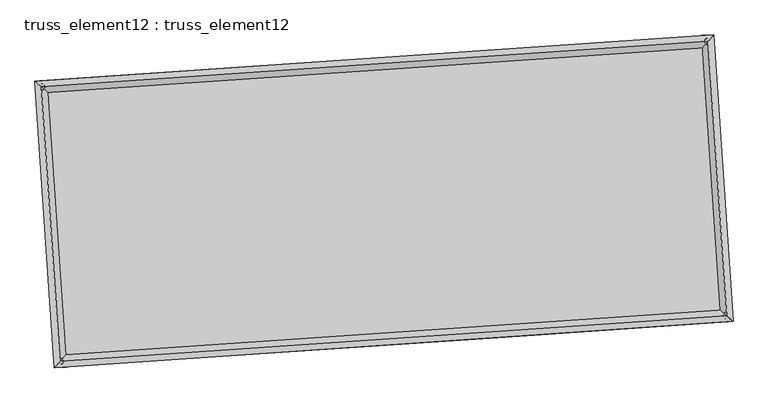
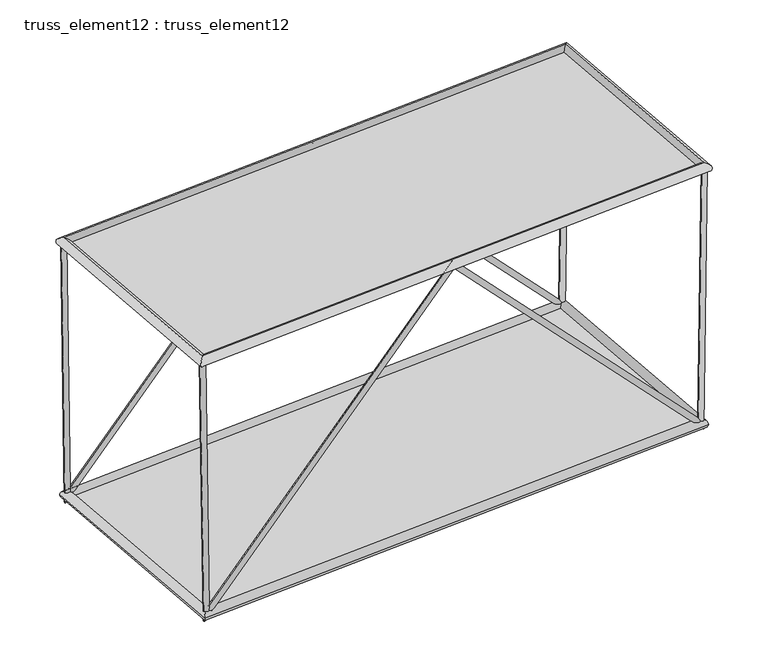
"""IFC4 building model written with IfcOpenShell, lengths in millimetres: plate geometry, truss_element12 : truss_element12."""

import ifcopenshell
import ifcopenshell.guid

model = None  # the IFC model being written
_history = None  # IfcOwnerHistory: only IFC2X3 demands one
_inside = {}  # id of a spatial element -> (the spatial element, [elements in it])
_under = {}  # id of a project, library or spatial element -> (it, [spatial elements below it])
_declared = {}  # id of a project -> (the project, [libraries it declares])
_typed = {}  # id of a type object -> (the type object, [elements of that type])
_made_of = {}  # id of a material, layer set ... -> (it, [elements and type objects made of it])


def new_model(schema):
    """Start an empty IFC model of exactly this schema.

    Asked for "IFC4X3", IfcOpenShell would pick the latest addendum, in which some entities
    have other attributes; the version numbers below select the first issue.
    IFC2X3 requires an IfcOwnerHistory on every rooted entity: one is made here for all.
    """
    global model, _history
    if schema == "IFC4X3":
        model = ifcopenshell.file(schema_version=(4, 3, 0, 0))
    else:
        model = ifcopenshell.file(schema=schema)
    _inside.clear()
    _under.clear()
    _declared.clear()
    _typed.clear()
    _made_of.clear()
    _history = None
    if model.schema == "IFC2X3":
        org = make("IfcOrganization", Name="unknown")
        user = make(
            "IfcPersonAndOrganization",
            ThePerson=make("IfcPerson", FamilyName="unknown"),
            TheOrganization=org,
        )
        app = make(
            "IfcApplication",
            ApplicationDeveloper=org,
            Version="unknown",
            ApplicationFullName="unknown",
            ApplicationIdentifier="unknown",
        )
        _history = make(
            "IfcOwnerHistory",
            OwningUser=user,
            OwningApplication=app,
            ChangeAction="ADDED",
            CreationDate=0,
        )
    return model


def make(cls, **values):
    """One entity of the class cls with the attributes given. An attribute that is None is left unset."""
    return model.create_entity(
        cls, **{name: value for name, value in values.items() if value is not None}
    )


def rooted(cls, **values):
    """An entity with a GlobalId (a new one), such as an element, a storey or a relation."""
    return make(cls, GlobalId=ifcopenshell.guid.new(), OwnerHistory=_history, **values)


def si_unit(unit_type, name, prefix=None):
    """IfcSIUnit, for example si_unit("LENGTHUNIT", "METRE", prefix="MILLI")."""
    return make("IfcSIUnit", UnitType=unit_type, Prefix=prefix, Name=name)


def assignment(units):
    """IfcUnitAssignment: the units of a project."""
    return None if units is None else make("IfcUnitAssignment", Units=units)


def point(xyz):
    """IfcCartesianPoint."""
    return None if xyz is None else make("IfcCartesianPoint", Coordinates=xyz)


def direction(xyz):
    """IfcDirection."""
    return None if xyz is None else make("IfcDirection", DirectionRatios=xyz)


def frame(location, z_axis=None, x_axis=None):
    """IfcAxis2Placement3D, a coordinate frame: its origin and axes. An axis left out is left unset."""
    return make(
        "IfcAxis2Placement3D",
        Location=point(location),
        Axis=direction(z_axis),
        RefDirection=direction(x_axis),
    )


def origin():
    """The frame at (0, 0, 0) with its axes left unset."""
    return frame((0.0, 0.0, 0.0))


def origin_with_axes():
    """The frame at (0, 0, 0) with the z axis (0, 0, 1) and the x axis (1, 0, 0) written out."""
    return frame((0.0, 0.0, 0.0), z_axis=(0.0, 0.0, 1.0), x_axis=(1.0, 0.0, 0.0))


def place(relative_to, where):
    """IfcLocalPlacement: puts the frame where relative to a parent placement (None: the world)."""
    return make(
        "IfcLocalPlacement", PlacementRelTo=relative_to, RelativePlacement=where
    )


def context(
    kind, dimensions, precision=None, world=None, true_north=None, identifier=None
):
    """IfcGeometricRepresentationContext, for example the 3D "Model" context."""
    return make(
        "IfcGeometricRepresentationContext",
        ContextIdentifier=identifier,
        ContextType=kind,
        CoordinateSpaceDimension=dimensions,
        Precision=precision,
        WorldCoordinateSystem=world,
        TrueNorth=true_north,
    )


def project(units=None, contexts=None):
    """IfcProject with its units and contexts."""
    return rooted(
        "IfcProject",
        Name="project",
        RepresentationContexts=contexts,
        UnitsInContext=assignment(units),
    )


def spatial(cls, under=None, at=None, **own):
    """A site, building, storey or space (cls), placed at a placement, below another one or the project."""
    s = rooted(cls, ObjectPlacement=at, **own)
    if under is not None:
        _under.setdefault(under.id(), (under, []))[1].append(s)
    return s


def polyline(points):
    """IfcPolyline through the points."""
    return make("IfcPolyline", Points=[point(p) for p in points])


def circle_curve(where, radius):
    """IfcCircle in the frame where."""
    return make("IfcCircle", Position=where, Radius=radius)


def ellipse_curve(where, semi_axis1, semi_axis2):
    """IfcEllipse in the frame where."""
    return make(
        "IfcEllipse", Position=where, SemiAxis1=semi_axis1, SemiAxis2=semi_axis2
    )


def outline(outer, holes=None, kind="AREA"):
    """IfcArbitraryClosedProfileDef: a profile drawn as a closed curve; with holes, ...WithVoids."""
    if holes is None:
        return make("IfcArbitraryClosedProfileDef", ProfileType=kind, OuterCurve=outer)
    return make(
        "IfcArbitraryProfileDefWithVoids",
        ProfileType=kind,
        OuterCurve=outer,
        InnerCurves=holes,
    )


def extrude(swept, where, along, depth):
    """IfcExtrudedAreaSolid: the profile swept, set in the frame where, extruded along a direction by depth."""
    return make(
        "IfcExtrudedAreaSolid",
        SweptArea=swept,
        Position=where,
        ExtrudedDirection=direction(along),
        Depth=depth,
    )


def shape(context_of_items, identifier, shape_type, items):
    """IfcShapeRepresentation: the items that make up one representation, for example the "Body"."""
    return make(
        "IfcShapeRepresentation",
        ContextOfItems=context_of_items,
        RepresentationIdentifier=identifier,
        RepresentationType=shape_type,
        Items=items,
    )


def source(mapping_origin, context_of_items, identifier, shape_type, items):
    """IfcRepresentationMap: a shape defined once, which mapped items show again and again."""
    return make(
        "IfcRepresentationMap",
        MappingOrigin=mapping_origin,
        MappedRepresentation=shape(context_of_items, identifier, shape_type, items),
    )


def transform(
    local_origin,
    x_axis=None,
    y_axis=None,
    z_axis=None,
    scale=None,
    scale2=None,
    scale3=None,
    uniform=True,
):
    """IfcCartesianTransformationOperator3D, or its non-uniform kind. x_axis, y_axis, z_axis: its Axis1, 2, 3."""
    if uniform:
        return make(
            "IfcCartesianTransformationOperator3D",
            Axis1=direction(x_axis),
            Axis2=direction(y_axis),
            LocalOrigin=point(local_origin),
            Scale=scale,
            Axis3=direction(z_axis),
        )
    return make(
        "IfcCartesianTransformationOperator3DnonUniform",
        Axis1=direction(x_axis),
        Axis2=direction(y_axis),
        LocalOrigin=point(local_origin),
        Scale=scale,
        Axis3=direction(z_axis),
        Scale2=scale2,
        Scale3=scale3,
    )


def mapped(mapping_source, mapping_target):
    """IfcMappedItem: shows the shape of a source again, moved by a transform."""
    return make(
        "IfcMappedItem", MappingSource=mapping_source, MappingTarget=mapping_target
    )


def made_of(thing, what):
    """Note that an element or type object is made of a material, layer set ...; save() writes the relation."""
    if what is not None:
        _made_of.setdefault(what.id(), (what, []))[1].append(thing)
    return thing


def element(
    cls,
    number,
    at=None,
    inside=None,
    cuts=None,
    type_object=None,
    material=None,
    context=None,
    identifier="Body",
    shape_type=None,
    held_by="IfcProductDefinitionShape",
    body=None,
    shapes=None,
    **own,
):
    """One element of the class cls, such as IfcWall. Its Tag is "e" and its number.

    at: its placement. inside: the storey or other place that contains it. cuts: it is an
    opening in that element (IfcRelVoidsElement). A single representation is given by context,
    identifier, shape_type and body (its items); several are given by shapes. held_by: the class
    of the entity that holds the representations. save() writes the other relations.
    """
    e = rooted(cls, Tag="e%d" % number, ObjectPlacement=at, **own)
    if body is not None:
        shapes = [shape(context, identifier, shape_type, body)]
    if shapes is not None:
        e.Representation = make(held_by, Representations=shapes)
    if inside is not None:
        _inside.setdefault(inside.id(), (inside, []))[1].append(e)
    if cuts is not None:
        rooted(
            "IfcRelVoidsElement", RelatingBuildingElement=cuts, RelatedOpeningElement=e
        )
    if type_object is not None:
        _typed.setdefault(type_object.id(), (type_object, []))[1].append(e)
    return made_of(e, material)


def aggregate(whole, parts):
    """IfcRelAggregates: a whole, such as a stair, and the parts it consists of."""
    return rooted("IfcRelAggregates", RelatingObject=whole, RelatedObjects=parts)


def save(model, path):
    """Write the relations noted so far, then the file.

    IfcRelAggregates (storeys below a building ...), IfcRelContainedInSpatialStructure (elements
    in a storey), IfcRelDefinesByType, IfcRelAssociatesMaterial and IfcRelDeclares: one each for
    every whole, place, type object, material and project.
    """
    for whole, parts in _under.values():
        aggregate(whole, parts)
    for where, things in _inside.values():
        rooted(
            "IfcRelContainedInSpatialStructure",
            RelatedElements=things,
            RelatingStructure=where,
        )
    for kind, things in _typed.values():
        rooted("IfcRelDefinesByType", RelatedObjects=things, RelatingType=kind)
    for what, things in _made_of.values():
        rooted("IfcRelAssociatesMaterial", RelatedObjects=things, RelatingMaterial=what)
    for by, libraries in _declared.values():
        rooted("IfcRelDeclares", RelatingContext=by, RelatedDefinitions=libraries)
    model.write(path)


def plane_surface(at):
    """IfcPlane: the flat surface through the origin of the frame at, square to its z axis."""
    return make("IfcPlane", Position=at)


def cylinder_surface(at, radius):
    """IfcCylindricalSurface: all points at the distance radius from the z axis of the frame at."""
    return make("IfcCylindricalSurface", Position=at, Radius=radius)


def advanced_brep(points, edges, surfaces, faces):
    """IfcAdvancedBrep: a solid bounded by faces that lie on surfaces and meet in shared edges.

    An edge is (start, end): straight between two places in points (the first is 0);
    or (start, end, curve); or (start, end, curve, False) where it runs against its curve.
    A face is (place in surfaces, loops), or (place, loops, False) where it looks against
    its surface's normal. A loop lists edges by number (the first is 1), with a minus sign
    where the edge is run from its end to its start. The first loop is the outer one.
    """
    corners = [point(p) for p in points]
    vertices = [make("IfcVertexPoint", VertexGeometry=c) for c in corners]
    made = []
    for start, end, *more in edges:
        made.append(
            make(
                "IfcEdgeCurve",
                EdgeStart=vertices[start],
                EdgeEnd=vertices[end],
                EdgeGeometry=more[0] if more else make("IfcPolyline", Points=[corners[start], corners[end]]),
                SameSense=more[1] if len(more) > 1 else True,
            )
        )
    hull = []
    for where, loops, *sense in faces:
        bounds = []
        for j, loop in enumerate(loops):
            ring = [make("IfcOrientedEdge", EdgeElement=made[abs(k) - 1], Orientation=k > 0) for k in loop]
            bounds.append(
                make(
                    "IfcFaceOuterBound" if j == 0 else "IfcFaceBound",
                    Bound=make("IfcEdgeLoop", EdgeList=ring),
                    Orientation=True,
                )
            )
        hull.append(make("IfcAdvancedFace", Bounds=bounds, FaceSurface=surfaces[where], SameSense=sense[0] if sense else True))
    return make("IfcAdvancedBrep", Outer=make("IfcClosedShell", CfsFaces=hull))


def truss_element12_truss_element12_be2aad90(model_context):
    return source(origin(), model_context, "Body", "SolidModel", [
        advanced_brep(
        [(-3735.6006401, 2271.406017, 5000.2050975), (-3834.6940161, 2258.0454232, 4998.791816), (-3666.6666291, 2276.1063651, 122.4057611), (-3762.3202537, 2262.980315, -122.4057611), (1063.0860418, 2598.6102203, 5071.6275519), (1063.5437029, 2592.0376334, 4927.3870537), (5794.0749811, 2921.1983719, 122.4145359), (5890.6859959, 2921.1821166, -122.4145359), (5861.782005, 2925.8150565, 5000.2102148), (5961.7721407, 2926.0292106, 4998.822083)],
        [
            (0, 1, circle_curve(frame((-3785.1473281, 2264.7257201, 4999.4984567), z_axis=(-0.014130777343730014, -0.0009635239909554328, 0.9998996913456774), x_axis=(-0.13360615268411807, 0.9910340686191066, -0.0009331672991190194)), 50.0)),
            (1, 0, circle_curve(frame((-3785.1473281, 2264.7257201, 4999.4984567), z_axis=(-0.014130777343730014, -0.0009635239909554328, 0.9998996913456774), x_axis=(-0.13360615268411807, 0.9910340686191066, -0.0009331672991190194)), 50.0)),
            (0, 2),
            (2, 3, ellipse_curve(frame((-3714.4934414, 2269.54334, 0.0), z_axis=(-0.9284028499826127, -0.06330426115068324, 0.366143030336955), x_axis=(0.3652948219557198, 0.024908065293541812, 0.9305585856546978)), 131.8265203, 50.0)),
            (3, 1),
            (3, 2, ellipse_curve(frame((-3714.4934414, 2269.54334, 0.0), z_axis=(-0.9284028499826127, -0.06330426115068324, 0.366143030336955), x_axis=(0.3652948219557198, 0.024908065293541812, 0.9305585856546978)), 131.8265203, 50.0)),
            (2, 4),
            (4, 5, ellipse_curve(frame((1063.3148723, 2595.3239268, 4999.5073028), z_axis=(-0.9976833939203528, -0.06802823808179481, -6.571949967975178e-05), x_axis=(6.556725362871375e-05, 4.470781780485672e-06, -0.9999999978404738)), 72.2772914, 50.0)),
            (5, 3),
            (5, 4, ellipse_curve(frame((1063.3148723, 2595.3239268, 4999.5073028), z_axis=(-0.9976833939203528, -0.06802823808179481, -6.571949967975178e-05), x_axis=(6.556725362871375e-05, 4.470781780485672e-06, -0.9999999978404738)), 72.2772914, 50.0)),
            (4, 6),
            (6, 7, ellipse_curve(frame((5842.3804885, 2921.1902443, 0.0), z_axis=(-0.9283327861344512, -0.06329948376321463, -0.36632146202912796), x_axis=(-0.3654728402923341, -0.024920203687204556, 0.9304883591194691)), 131.8459204, 50.0)),
            (7, 5),
            (7, 6, ellipse_curve(frame((5842.3804885, 2921.1902443, 0.0), z_axis=(-0.9283327861344512, -0.06329948376321463, -0.36632146202912796), x_axis=(-0.3654728402923341, -0.024920203687204556, 0.9304883591194691)), 131.8459204, 50.0)),
            (8, 9, circle_curve(frame((5911.7770728, 2925.9221335, 4999.5161489), z_axis=(0.013879316866173963, 0.0009463778568815537, 0.9999032297839028), x_axis=(-0.0021544712619485026, 0.9999972590806624, -0.0009165613694543245)), 50.0)),
            (9, 8, circle_curve(frame((5911.7770728, 2925.9221335, 4999.5161489), z_axis=(0.013879316866173963, 0.0009463778568815537, 0.9999032297839028), x_axis=(-0.0021544712619485026, 0.9999972590806624, -0.0009165613694543245)), 50.0)),
            (6, 8),
            (9, 7),
        ],
        [
            plane_surface(frame((-3785.1473281, 2314.7256969, 4999.5466377), z_axis=(-0.01413077734373192, -0.0009635239909557289, 0.9998996913456774), x_axis=(0.9999001555813771, -1.3616702533525423e-05, 0.014130770783065568))),
            cylinder_surface(frame((-3785.1473281, 2264.7257201, 4999.4984567), z_axis=(-0.014130777343730014, -0.0009635239909554328, 0.9998996913456774), x_axis=(-0.13360615268411807, 0.9910340686191066, -0.0009331672991190194)), 50.0),
            cylinder_surface(frame((-3714.4934414, 2269.54334, 0.0), z_axis=(-0.6901302832567465, -0.04705736058446858, -0.7221535826586936), x_axis=(-0.020411599373552875, 0.9987523749165735, -0.04557477602268607)), 50.0),
            cylinder_surface(frame((1063.3148723, 2595.3239268, 4999.5073028), z_axis=(-0.6902249765493501, -0.04706381736012831, 0.7220626557598319), x_axis=(-0.11534328032643532, 0.9922793444614997, -0.045581029371808676)), 50.0),
            plane_surface(frame((5911.7770728, 2875.9221559, 4999.5634724), z_axis=(0.013879316866172038, 0.000946377856885389, 0.9999032297839029), x_axis=(0.999903677642666, -1.3136343474329222e-05, -0.013879310649599559))),
            cylinder_surface(frame((5842.3804885, 2921.1902443, 0.0), z_axis=(-0.013879316866173963, -0.0009463778568815537, -0.9999032297839028), x_axis=(-0.0021544712619485026, 0.9999972590806624, -0.0009165613694543245)), 50.0),
        ],
        [
            (0, [[1, 2]]),
            (1, [[-1, 3, 4, 5]]),
            (1, [[-2, -5, 6, -3]]),
            (2, [[-4, 7, 8, 9]]),
            (2, [[-6, -9, 10, -7]]),
            (3, [[-8, 11, 12, 13]]),
            (3, [[-10, -13, 14, -11]]),
            (4, [[15, 16]]),
            (5, [[-12, 17, -16, 18]]),
            (5, [[-14, -18, -15, -17]]),
        ],
    ),
        advanced_brep(
        [(-3463.4876872, -1719.3275673, 5000.2050975), (-3562.5810632, -1732.6881611, 4998.791816), (-3394.5536762, -1714.6272192, 122.4057611), (-3490.2073008, -1727.7532693, -122.4057611), (1335.1989947, -1392.123364, 5071.6275519), (1335.6566558, -1398.6959509, 4927.3870537), (6066.1879341, -1069.5352124, 122.4145359), (6162.7989488, -1069.5514677, -122.4145359), (6133.8949579, -1064.9185278, 5000.2102148), (6233.8850936, -1064.7043737, 4998.822083)],
        [
            (0, 1, circle_curve(frame((-3513.0343752, -1726.0078642, 4999.4984567), z_axis=(-0.014130777343729955, -0.000963523990955448, 0.9998996913456774), x_axis=(-0.13360615268411774, 0.9910340686191066, -0.0009331672991189919)), 50.0)),
            (1, 0, circle_curve(frame((-3513.0343752, -1726.0078642, 4999.4984567), z_axis=(-0.014130777343729955, -0.000963523990955448, 0.9998996913456774), x_axis=(-0.13360615268411774, 0.9910340686191066, -0.0009331672991189919)), 50.0)),
            (0, 2),
            (2, 3, ellipse_curve(frame((-3442.3804885, -1721.1902443, 0.0), z_axis=(-0.9284028499826127, -0.06330426115068316, 0.3661430303369552), x_axis=(0.36529482195571994, 0.024908065293541774, 0.9305585856546977)), 131.8265203, 50.0)),
            (3, 1),
            (3, 2, ellipse_curve(frame((-3442.3804885, -1721.1902443, 0.0), z_axis=(-0.9284028499826127, -0.06330426115068316, 0.3661430303369552), x_axis=(0.36529482195571994, 0.024908065293541774, 0.9305585856546977)), 131.8265203, 50.0)),
            (2, 4),
            (4, 5, ellipse_curve(frame((1335.4278253, -1395.4096575, 4999.5073028), z_axis=(-0.9976833939203528, -0.06802823808179471, -6.571949967999249e-05), x_axis=(6.556725362902129e-05, 4.470781780543329e-06, -0.9999999978404738)), 72.2772914, 50.0)),
            (5, 3),
            (5, 4, ellipse_curve(frame((1335.4278253, -1395.4096575, 4999.5073028), z_axis=(-0.9976833939203528, -0.06802823808179471, -6.571949967999249e-05), x_axis=(6.556725362902129e-05, 4.470781780543329e-06, -0.9999999978404738)), 72.2772914, 50.0)),
            (4, 6),
            (6, 7, ellipse_curve(frame((6114.4934414, -1069.54334, 0.0), z_axis=(-0.9283327861344511, -0.0632994837632146, -0.3663214620291284), x_axis=(-0.3654728402923345, -0.024920203687204566, 0.9304883591194689)), 131.8459204, 50.0)),
            (7, 5),
            (7, 6, ellipse_curve(frame((6114.4934414, -1069.54334, 0.0), z_axis=(-0.9283327861344511, -0.0632994837632146, -0.3663214620291284), x_axis=(-0.3654728402923345, -0.024920203687204566, 0.9304883591194689)), 131.8459204, 50.0)),
            (8, 9, circle_curve(frame((6183.8900257, -1064.8114508, 4999.5161489), z_axis=(0.013879316866173474, 0.0009463778568815351, 0.9999032297839028), x_axis=(-0.0021544712619487186, 0.9999972590806624, -0.000916561369454304)), 50.0)),
            (9, 8, circle_curve(frame((6183.8900257, -1064.8114508, 4999.5161489), z_axis=(0.013879316866173474, 0.0009463778568815351, 0.9999032297839028), x_axis=(-0.0021544712619487186, 0.9999972590806624, -0.000916561369454304)), 50.0)),
            (6, 8),
            (9, 7),
        ],
        [
            plane_surface(frame((-3513.0343752, -1676.0078874, 4999.5466377), z_axis=(-0.01413077734373192, -0.0009635239909557289, 0.9998996913456774), x_axis=(0.9999001555813771, -1.3616702533525423e-05, 0.014130770783065568))),
            cylinder_surface(frame((-3513.0343752, -1726.0078642, 4999.4984567), z_axis=(-0.014130777343729955, -0.000963523990955448, 0.9998996913456774), x_axis=(-0.13360615268411774, 0.9910340686191066, -0.0009331672991189919)), 50.0),
            cylinder_surface(frame((-3442.3804885, -1721.1902443, 0.0), z_axis=(-0.6901302832567464, -0.047057360584468466, -0.7221535826586933), x_axis=(-0.020411599373552827, 0.9987523749165735, -0.04557477602268599)), 50.0),
            cylinder_surface(frame((1335.4278253, -1395.4096575, 4999.5073028), z_axis=(-0.6902249765493508, -0.04706381736012834, 0.7220626557598315), x_axis=(-0.11534328032643515, 0.9922793444614998, -0.045581029371808586)), 50.0),
            plane_surface(frame((6183.8900257, -1114.8114284, 4999.5634724), z_axis=(0.013879316866172038, 0.0009463778568853864, 0.9999032297839029), x_axis=(0.999903677642666, -1.3136343474329222e-05, -0.013879310649599559))),
            cylinder_surface(frame((6114.4934414, -1069.54334, 0.0), z_axis=(-0.013879316866173474, -0.0009463778568815351, -0.9999032297839028), x_axis=(-0.0021544712619487186, 0.9999972590806624, -0.000916561369454304)), 50.0),
        ],
        [
            (0, [[1, 2]]),
            (1, [[-1, 3, 4, 5]]),
            (1, [[-2, -5, 6, -3]]),
            (2, [[-4, 7, 8, 9]]),
            (2, [[-6, -9, 10, -7]]),
            (3, [[-8, 11, 12, 13]]),
            (3, [[-10, -13, 14, -11]]),
            (4, [[15, 16]]),
            (5, [[-12, 17, -16, 18]]),
            (5, [[-14, -18, -15, -17]]),
        ],
    ),
        advanced_brep(
        [(-3513.0297394, -1726.0027261, 4909.4984569), (-3513.0390111, -1726.0130023, 5089.4984566), (-3785.1526185, 2264.7301814, 5089.4984566), (-3785.1420377, 2264.7212588, 4909.4984569), (5911.7813818, 2925.9272494, 5089.5161488), (5911.7727639, 2925.9170177, 4909.516149), (6183.8949893, -1064.8159343, 5089.5161488), (6183.8850622, -1064.8069672, 4909.516149)],
        [
            (0, 1, ellipse_curve(frame((-3513.0343752, -1726.0078642, 4999.4984567), z_axis=(-0.7535719234042865, 0.6573654662781635, -1.2871387339014257e-06), x_axis=(-0.657365466276915, -0.7535719234053757, -1.287138733901674e-06)), 127.2792206, 90.0)),
            (1, 2),
            (2, 3, ellipse_curve(frame((-3785.1473281, 2264.7257201, 4999.4984567), z_axis=(-0.657365466276915, -0.7535719234053756, -1.287138733901906e-06), x_axis=(0.7535719234042865, -0.6573654662781635, 1.2871387339016578e-06)), 127.2792206, 90.0)),
            (3, 0),
            (1, 0, ellipse_curve(frame((-3513.0343752, -1726.0078642, 4999.4984567), z_axis=(-0.7535719234042865, 0.6573654662781635, -1.2871387339014257e-06), x_axis=(-0.657365466276915, -0.7535719234053757, -1.287138733901674e-06)), 127.2792206, 90.0)),
            (3, 2, ellipse_curve(frame((-3785.1473281, 2264.7257201, 4999.4984567), z_axis=(-0.657365466276915, -0.7535719234053756, -1.287138733901906e-06), x_axis=(0.7535719234042865, -0.6573654662781635, 1.2871387339016578e-06)), 127.2792206, 90.0)),
            (2, 4),
            (4, 5, ellipse_curve(frame((5911.7770728, 2925.9221335, 4999.5161489), z_axis=(-0.7535719234042866, 0.6573654662781635, -1.2871387339018918e-06), x_axis=(-0.657365466276915, -0.7535719234053757, -1.2871387339016724e-06)), 127.2792206, 90.0)),
            (5, 3),
            (5, 4, ellipse_curve(frame((5911.7770728, 2925.9221335, 4999.5161489), z_axis=(-0.7535719234042866, 0.6573654662781635, -1.2871387339018918e-06), x_axis=(-0.657365466276915, -0.7535719234053757, -1.2871387339016724e-06)), 127.2792206, 90.0)),
            (4, 6),
            (6, 7, ellipse_curve(frame((6183.8900257, -1064.8114508, 4999.5161489), z_axis=(0.6573654662769151, 0.7535719234053756, 1.2871387339014406e-06), x_axis=(-0.7535719234042866, 0.6573654662781636, -1.2871387339016595e-06)), 127.2792206, 90.0)),
            (7, 5),
            (7, 6, ellipse_curve(frame((6183.8900257, -1064.8114508, 4999.5161489), z_axis=(0.6573654662769151, 0.7535719234053756, 1.2871387339014406e-06), x_axis=(-0.7535719234042866, 0.6573654662781636, -1.2871387339016595e-06)), 127.2792206, 90.0)),
            (6, 1),
            (0, 7),
        ],
        [
            cylinder_surface(frame((-3513.0343752, -1726.0078642, 4999.4984567), z_axis=(0.0680282382286971, -0.9976833960748769, 0.0), x_axis=(-0.9976833945508087, -0.06802823812477667, -5.5273991684341074e-05)), 90.0),
            cylinder_surface(frame((-3785.1473281, 2264.7257201, 4999.4984567), z_axis=(-0.997683396073224, -0.06802823822858504, -1.8202890541396347e-06), x_axis=(-0.06802823803443349, 0.9976833946561565, -5.3453702632802165e-05)), 90.0),
            cylinder_surface(frame((5911.7770728, 2925.9221335, 4999.5161489), z_axis=(-0.06802823822869682, 0.997683396074877, 0.0), x_axis=(0.9976833947449603, 0.06802823813801485, -5.1633413581263256e-05)), 90.0),
            cylinder_surface(frame((6183.8900257, -1064.8114508, 4999.5161489), z_axis=(0.997683396073224, 0.06802823822858474, 1.8202890541393063e-06), x_axis=(0.06802823822858474, -0.9976833946429181, -5.345370263280218e-05)), 90.0),
        ],
        [
            (0, [[1, 2, 3, 4]]),
            (0, [[5, -4, 6, -2]]),
            (1, [[-3, 7, 8, 9]]),
            (1, [[-6, -9, 10, -7]]),
            (2, [[-8, 11, 12, 13]]),
            (2, [[-10, -13, 14, -11]]),
            (3, [[-12, 15, -1, 16]]),
            (3, [[-14, -16, -5, -15]]),
        ],
    ),
        advanced_brep(
        [(-3358.7115243, -1625.2761972, 0.0), (-3526.0494527, -1817.1042913, 0.0), (-3810.4074885, 2353.2123043, 0.0), (-3618.5793943, 2185.8743758, 0.0), (5926.0494527, 3017.1042913, 0.0), (5758.7115243, 2825.2761972, 0.0), (6210.4074885, -1153.2123043, 0.0), (6018.5793943, -985.8743758, 0.0)],
        [
            (0, 1, ellipse_curve(frame((-3442.3804885, -1721.1902443, 0.0), z_axis=(-0.7535719234054593, 0.6573654662780791, 0.0), x_axis=(-0.6573654662780791, -0.7535719234054594, 0.0)), 127.2792206, 90.0)),
            (1, 2),
            (2, 3, ellipse_curve(frame((-3714.4934414, 2269.54334, 0.0), z_axis=(-0.6573654662780791, -0.7535719234054593, 0.0), x_axis=(0.7535719234054593, -0.6573654662780793, 0.0)), 127.2792206, 90.0)),
            (3, 0),
            (1, 0, ellipse_curve(frame((-3442.3804885, -1721.1902443, 0.0), z_axis=(-0.7535719234054593, 0.6573654662780791, 0.0), x_axis=(-0.6573654662780791, -0.7535719234054594, 0.0)), 127.2792206, 90.0)),
            (3, 2, ellipse_curve(frame((-3714.4934414, 2269.54334, 0.0), z_axis=(-0.6573654662780791, -0.7535719234054593, 0.0), x_axis=(0.7535719234054593, -0.6573654662780793, 0.0)), 127.2792206, 90.0)),
            (2, 4),
            (4, 5, ellipse_curve(frame((5842.3804885, 2921.1902443, 0.0), z_axis=(-0.7535719234054593, 0.6573654662780792, 0.0), x_axis=(-0.6573654662780793, -0.7535719234054592, 0.0)), 127.2792206, 90.0)),
            (5, 3),
            (5, 4, ellipse_curve(frame((5842.3804885, 2921.1902443, 0.0), z_axis=(-0.7535719234054593, 0.6573654662780792, 0.0), x_axis=(-0.6573654662780793, -0.7535719234054592, 0.0)), 127.2792206, 90.0)),
            (4, 6),
            (6, 7, ellipse_curve(frame((6114.4934414, -1069.54334, 0.0), z_axis=(0.6573654662780793, 0.7535719234054593, 0.0), x_axis=(-0.7535719234054594, 0.6573654662780792, 0.0)), 127.2792206, 90.0)),
            (7, 5),
            (7, 6, ellipse_curve(frame((6114.4934414, -1069.54334, 0.0), z_axis=(0.6573654662780793, 0.7535719234054593, 0.0), x_axis=(-0.7535719234054594, 0.6573654662780792, 0.0)), 127.2792206, 90.0)),
            (6, 1),
            (0, 7),
        ],
        [
            cylinder_surface(frame((-3442.3804885, -1721.1902443, 0.0), z_axis=(0.06802823822870308, -0.9976833960748764, 0.0), x_axis=(-0.9976833960748764, -0.06802823822870308, 0.0)), 90.0),
            cylinder_surface(frame((-3714.4934414, 2269.54334, 0.0), z_axis=(-0.9976833960748764, -0.06802823822870367, 0.0), x_axis=(-0.06802823822870367, 0.9976833960748764, 0.0)), 90.0),
            cylinder_surface(frame((5842.3804885, 2921.1902443, 0.0), z_axis=(-0.06802823822870292, 0.9976833960748764, 0.0), x_axis=(0.9976833960748764, 0.06802823822870292, 0.0)), 90.0),
            cylinder_surface(frame((6114.4934414, -1069.54334, 0.0), z_axis=(0.9976833960748764, 0.0680282382287036, 0.0), x_axis=(0.0680282382287036, -0.9976833960748764, 0.0)), 90.0),
        ],
        [
            (0, [[1, 2, 3, 4]]),
            (0, [[5, -4, 6, -2]]),
            (1, [[-3, 7, 8, 9]]),
            (1, [[-6, -9, 10, -7]]),
            (2, [[-8, 11, 12, 13]]),
            (2, [[-10, -13, 14, -11]]),
            (3, [[-12, 15, -1, 16]]),
            (3, [[-14, -16, -5, -15]]),
        ],
    ),
        extrude(outline(polyline([(-3442.3804885, -1721.1902443), (-3714.4934414, 2269.54334), (5842.3804885, 2921.1902443), (6114.4934414, -1069.54334), (-3442.3804885, -1721.1902443)])), origin_with_axes(), (0.0, 0.0, 1.0), 20.0),
        extrude(outline(polyline([(-2000.0, 4859.7202475), (2000.0, 4859.7202475), (1999.9999999, -4859.7202475), (-2000.0000001, -4859.7202474), (-2000.0, 4859.7202475)])), frame((1199.3713488, 599.9571347, 4999.5073028), z_axis=(-1.816072165371791e-06, -1.2383105742010014e-07, 0.9999999999983433), x_axis=(-0.06802823822870292, 0.9976833960748764, 0.0)), (0.0, 0.0, 1.0), 20.0),
    ])


if __name__ == "__main__":
    model = new_model("IFC4")
    model_context = context("Model", 3, world=origin())
    ifc_project = project(units=[si_unit("LENGTHUNIT", "METRE", prefix="MILLI")], contexts=[model_context])
    site = spatial("IfcSite", under=ifc_project)
    building = spatial("IfcBuilding", under=site)
    placement = place(None, origin())
    truss_element12_truss_element12_shape = truss_element12_truss_element12_be2aad90(model_context)
    element("IfcPlate", 1, ObjectType="truss_element12 : truss_element12", at=placement, inside=building, context=model_context, shape_type="MappedRepresentation", body=[
        mapped(truss_element12_truss_element12_shape, transform((0.0, 0.0, 0.0), x_axis=(1.0, 0.0, 0.0), y_axis=(0.0, 1.0, 0.0), z_axis=(0.0, 0.0, 1.0))),
    ])
    save(model, "model.ifc")

# Revit data of these elements
# Type "truss_element12 : truss_element12"
#   steellbar1 = 90 mm
#   steelbar2 = 50 mm
#   offset1 = 5000 mm
#   M = Default Roof
# Element 1 (IfcPlate, "truss_element12 : truss_element12")
#   Materials on its faces: "Default Roof"
# Materials
#   "Default Roof": class "Miscellaneous", colour RGB 0 127 0, transparency 0, Comments = "Rendering appearance not upgraded Rendering appearance not upgraded ", Cost = 0
